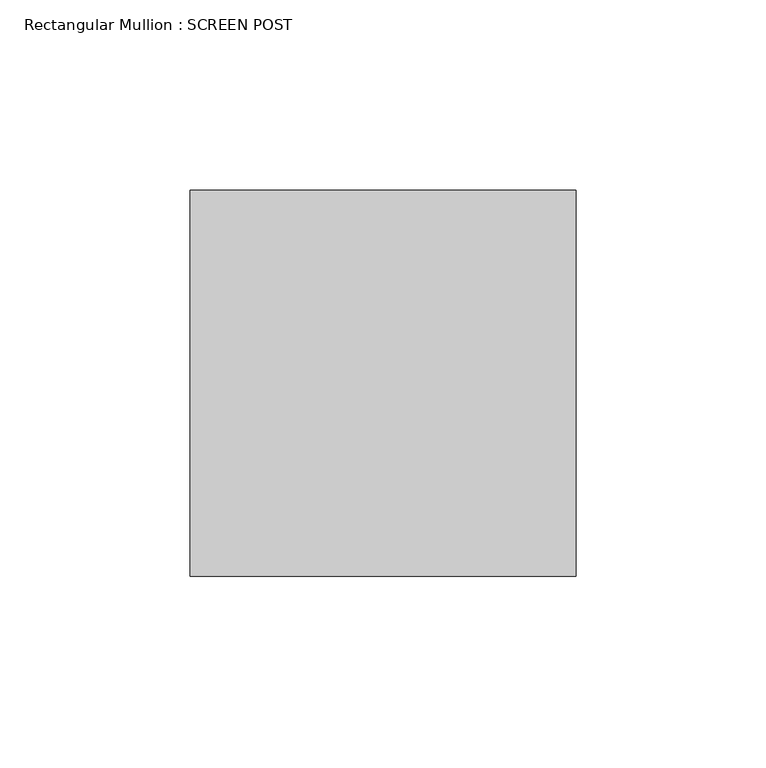
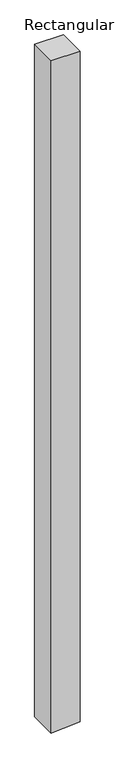
"""IFC4 building model written with IfcOpenShell, lengths in millimetres: member geometry, Rectangular Mullion : SCREEN POST."""

from ifc_helpers import new_model, si_unit, frame, origin, place, context, project, spatial, polyline, outline, extrude, source, transform, mapped, element, save


def rectangular_mullion_screen_post_24edb84c(model_context):
    return source(origin(), model_context, "Body", "SweptSolid", [
        extrude(outline(polyline([(0.0, 50.8), (0.0, -50.8), (-2520.3252536, -50.8), (-2517.5463557, -6.3376339), (-2513.9752536, 50.8), (0.0, 50.8)])), frame((0.0, -50.8, 0.0), z_axis=(0.0, 1.0, 0.0), x_axis=(0.0, 0.0, 1.0)), (0.0, 0.0, 1.0), 101.6),
    ])


if __name__ == "__main__":
    model = new_model("IFC4")
    model_context = context("Model", 3, world=origin())
    ifc_project = project(units=[si_unit("LENGTHUNIT", "METRE", prefix="MILLI")], contexts=[model_context])
    site = spatial("IfcSite", under=ifc_project)
    building = spatial("IfcBuilding", under=site)
    placement = place(None, origin())
    rectangular_mullion_screen_post_shape = rectangular_mullion_screen_post_24edb84c(model_context)
    element("IfcMember", 1, ObjectType="Rectangular Mullion : SCREEN POST", at=placement, inside=building, context=model_context, shape_type="MappedRepresentation", body=[
        mapped(rectangular_mullion_screen_post_shape, transform((0.0, 0.0, 0.0), x_axis=(1.0, 0.0, 0.0), y_axis=(0.0, 1.0, 0.0), z_axis=(0.0, 0.0, 1.0))),
    ])
    save(model, "model.ifc")

# Revit data of these elements
# Type "Rectangular Mullion : SCREEN POST"
#   built-in parameter 1007304 = 0.333333 (stored number, unit not read)
#   built-in parameter 1007301 = 0.166667 (stored number, unit not read)
#   built-in parameter 1007300 = 0.166667 (stored number, unit not read)
# Element 1 (IfcMember, "Rectangular Mullion : SCREEN POST")
#   Materials on its faces: "GLULAMS COLUMNS\n(PRESSURE TREATED W/ PENTA IN SOLVENT) (EXTERIOR STAIN: PENOFIN VERDE EXT. STAIN - COLOR: CEDAR)"
# Materials
#   "GLULAMS COLUMNS\n(PRESSURE TREATED W/ PENTA IN SOLVENT) (EXTERIOR STAIN: PENOFIN VERDE EXT. STAIN - COLOR: CEDAR)": class "Wood", colour RGB 164 134 123, transparency 0, Description = "Pinus Echinata", Cost = 0
